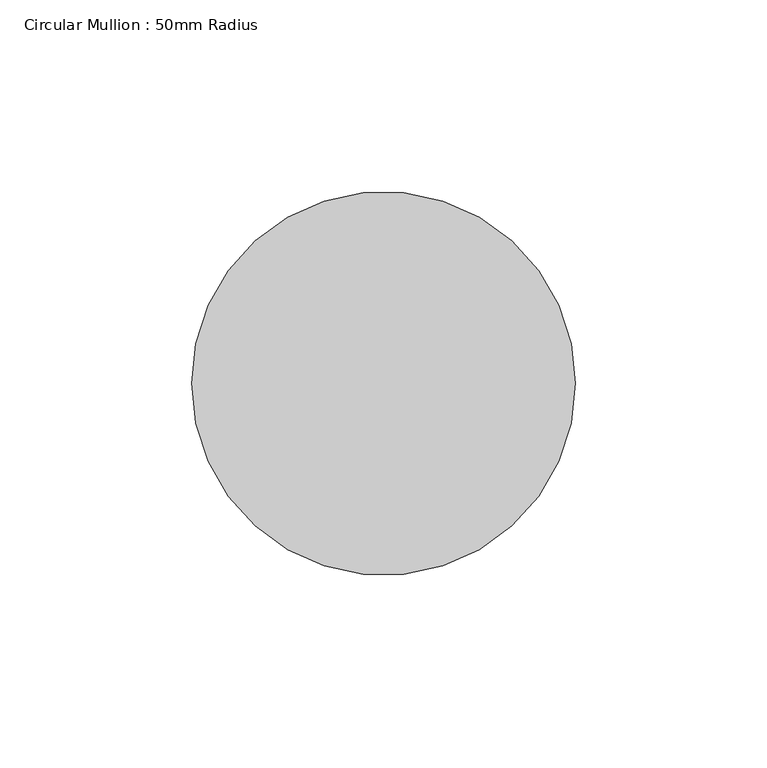
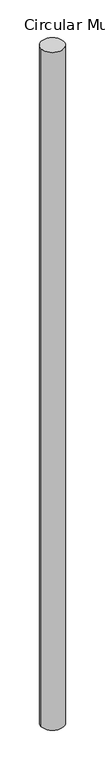
"""IFC4 building model written with IfcOpenShell, lengths in millimetres: member geometry, Circular Mullion : 50mm Radius."""

from ifc_helpers import new_model, si_unit, point, frame, frame_2d, origin, place, context, project, spatial, circle_curve, trimmed, segment, composite_curve, outline, extrude, source, transform, mapped, element, save


def circular_mullion_50mm_radius_24ec511a(model_context):
    return source(origin(), model_context, "Body", "SweptSolid", [
        extrude(outline(composite_curve([segment(trimmed(circle_curve(frame_2d((-50.0, 0.0)), 50.0), [point((0.0, 0.0))], [point((-100.0, 0.0))], False, "CARTESIAN"), True, "CONTINUOUS"), segment(trimmed(circle_curve(frame_2d((-50.0, 0.0)), 50.0), [point((-100.0, 0.0))], [point((0.0, 0.0))], False, "CARTESIAN"), True, "CONTINUOUS")], self_intersect=False)), frame((0.0, 0.0, -3175.7913192), z_axis=(0.0, 0.0, 1.0), x_axis=(1.0, 0.0, 0.0)), (0.0, 0.0, 1.0), 3175.7913192),
    ])


if __name__ == "__main__":
    model = new_model("IFC4")
    model_context = context("Model", 3, world=origin())
    ifc_project = project(units=[si_unit("LENGTHUNIT", "METRE", prefix="MILLI")], contexts=[model_context])
    site = spatial("IfcSite", under=ifc_project)
    building = spatial("IfcBuilding", under=site)
    placement = place(None, origin())
    circular_mullion_50mm_radius_shape = circular_mullion_50mm_radius_24ec511a(model_context)
    element("IfcMember", 1, ObjectType="Circular Mullion : 50mm Radius", at=placement, inside=building, context=model_context, shape_type="MappedRepresentation", body=[
        mapped(circular_mullion_50mm_radius_shape, transform((0.0, 0.0, 0.0), x_axis=(1.0, 0.0, 0.0), y_axis=(0.0, 1.0, 0.0), z_axis=(0.0, 0.0, 1.0))),
    ])
    save(model, "model.ifc")

# Revit data of these elements
# Type "Circular Mullion : 50mm Radius"
#   built-in parameter 1007350 = 0.164042 (stored number, unit not read)
# Element 1 (IfcMember, "Circular Mullion : 50mm Radius")
#   Materials on its faces: "Aluminium"
# Materials
#   "Aluminium": class "Metal", colour RGB 247 247 247, transparency 0, Description = "Aluminium 6061", Cost = 0
